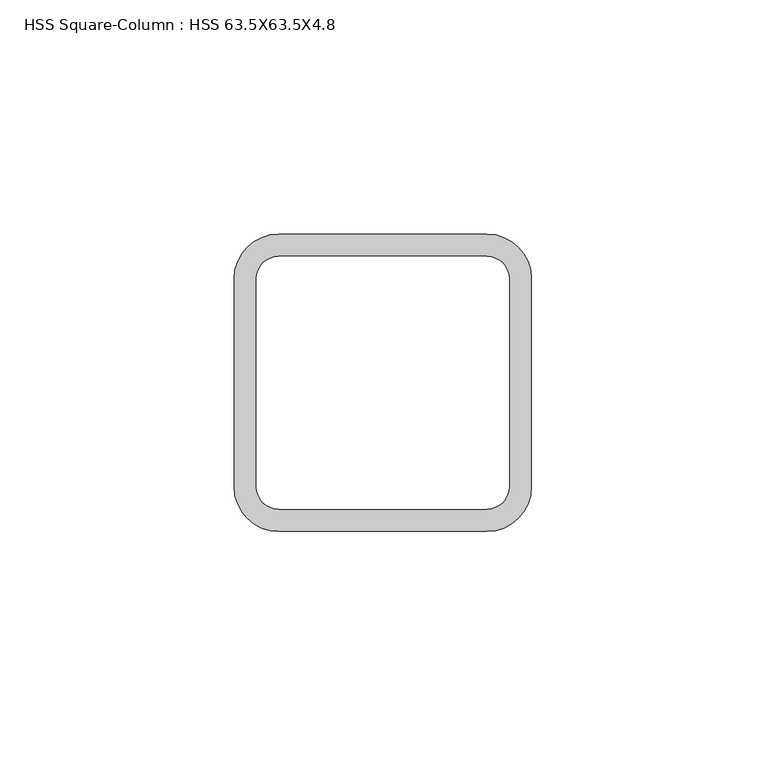
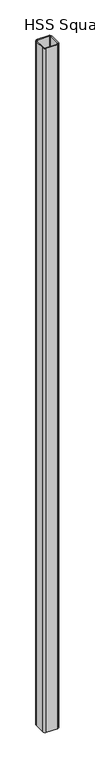
"""IFC4 building model written with IfcOpenShell, lengths in millimetres: column geometry, HSS Square-Column : HSS 63.5X63.5X4.8."""

from ifc_helpers import new_model, si_unit, point, frame, frame_2d, origin, place, context, project, spatial, polyline, circle_curve, trimmed, segment, composite_curve, outline, extrude, source, transform, mapped, element, save


def hss_square_column_hss_63_5x63_5x4_8_14cbe1c5(model_context):
    return source(origin(), model_context, "Body", "SweptSolid", [
        extrude(outline(composite_curve([segment(trimmed(circle_curve(frame_2d((22.225, 22.225)), 9.525), [point((22.225, 31.75))], [point((31.75, 22.225))], False, "CARTESIAN"), True, "CONTINUOUS"), segment(polyline([(31.75, 22.225), (31.75, -22.225)]), True, "CONTINUOUS"), segment(trimmed(circle_curve(frame_2d((22.225, -22.225)), 9.525), [point((31.75, -22.225))], [point((22.225, -31.75))], False, "CARTESIAN"), True, "CONTINUOUS"), segment(polyline([(22.225, -31.75), (-22.225, -31.75)]), True, "CONTINUOUS"), segment(trimmed(circle_curve(frame_2d((-22.225, -22.225)), 9.525), [point((-22.225, -31.75))], [point((-31.75, -22.225))], False, "CARTESIAN"), True, "CONTINUOUS"), segment(polyline([(-31.75, -22.225), (-31.75, 22.225)]), True, "CONTINUOUS"), segment(trimmed(circle_curve(frame_2d((-22.225, 22.225)), 9.525), [point((-31.75, 22.225))], [point((-22.225, 31.75))], False, "CARTESIAN"), True, "CONTINUOUS"), segment(polyline([(-22.225, 31.75), (22.225, 31.75)]), True, "CONTINUOUS")], self_intersect=False), holes=[composite_curve([segment(polyline([(22.225, 26.9875), (-22.225, 26.9875)]), True, "CONTINUOUS"), segment(trimmed(circle_curve(frame_2d((-22.225, 22.225)), 4.7625), [point((-22.225, 26.9875))], [point((-26.9875, 22.225))], True, "CARTESIAN"), True, "CONTINUOUS"), segment(polyline([(-26.9875, 22.225), (-26.9875, -22.225)]), True, "CONTINUOUS"), segment(trimmed(circle_curve(frame_2d((-22.225, -22.225)), 4.7625), [point((-26.9875, -22.225))], [point((-22.225, -26.9875))], True, "CARTESIAN"), True, "CONTINUOUS"), segment(polyline([(-22.225, -26.9875), (22.225, -26.9875)]), True, "CONTINUOUS"), segment(trimmed(circle_curve(frame_2d((22.225, -22.225)), 4.7625), [point((22.225, -26.9875))], [point((26.9875, -22.225))], True, "CARTESIAN"), True, "CONTINUOUS"), segment(polyline([(26.9875, -22.225), (26.9875, 22.225)]), True, "CONTINUOUS"), segment(trimmed(circle_curve(frame_2d((22.225, 22.225)), 4.7625), [point((26.9875, 22.225))], [point((22.225, 26.9875))], True, "CARTESIAN"), True, "CONTINUOUS")], self_intersect=False)]), frame((0.0, 0.0, 6240.0), z_axis=(0.0, 0.0, 1.0), x_axis=(1.0, 0.0, 0.0)), (0.0, 0.0, 1.0), 2900.0),
    ])


if __name__ == "__main__":
    model = new_model("IFC4")
    model_context = context("Model", 3, world=origin())
    ifc_project = project(units=[si_unit("LENGTHUNIT", "METRE", prefix="MILLI")], contexts=[model_context])
    site = spatial("IfcSite", under=ifc_project)
    building = spatial("IfcBuilding", under=site)
    placement = place(None, origin())
    hss_square_column_hss_63_5x63_5x4_8_shape = hss_square_column_hss_63_5x63_5x4_8_14cbe1c5(model_context)
    element("IfcColumn", 1, ObjectType="HSS Square-Column : HSS 63.5X63.5X4.8", at=placement, inside=building, context=model_context, shape_type="MappedRepresentation", body=[
        mapped(hss_square_column_hss_63_5x63_5x4_8_shape, transform((0.0, 0.0, 0.0), x_axis=(1.0, 0.0, 0.0), y_axis=(0.0, 1.0, 0.0), z_axis=(0.0, 0.0, 1.0))),
    ])
    save(model, "model.ifc")

# Revit data of these elements
# Type "HSS Square-Column : HSS 63.5X63.5X4.8"
#   Section Name Key = "HSS 2 1/2X2 1/2X3/16"
#   Assembly Code = "B10"
#   Width = 6.35 cm
#   Wall Nominal Thickness = 0.4763 cm
#   Wall Design Thickness = 0.442 cm
#   Torsional Moment of Inertia = 93.6521 cm⁴
#   Torsional Modulus = 30.4799 cm³
#   Section Area = 9.93546 cm²
#   Plastic Modulus weak axis = 21.6309 cm³
#   Plastic Modulus strong axis = 21.6309 cm³
#   Outer Fillet = 0.9525 cm
#   Nominal Weight = 8.31884 kgf/m
#   Moment of Inertia weak axis = 56.1912 cm⁴
#   Moment of Inertia strong axis = 56.1912 cm⁴
#   Inner Fillet = 0.4763 cm
#   Height = 6.35 cm
#   Elastic Modulus weak axis = 17.698 cm³
#   Elastic Modulus strong axis = 17.698 cm³
#   Centroid Vertical = 3.175 cm
#   Centroid Horizontal = 3.175 cm
#   Structural Material [instance default] = Steel ASTM A500, Grade B, Rectangular and Square
#   Principal Axes Angle = 0
# Element 1 (IfcColumn, "HSS Square-Column : HSS 63.5X63.5X4.8")
#   Structural Material = none
# Materials
#   "Steel ASTM A500, Grade B, Rectangular and Square": class "Metal", colour RGB 199 199 199, transparency 0, Description = "Carbon steel", Cost = 0
